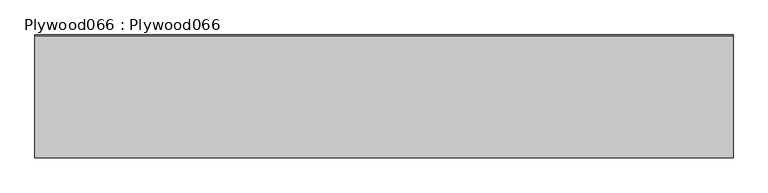
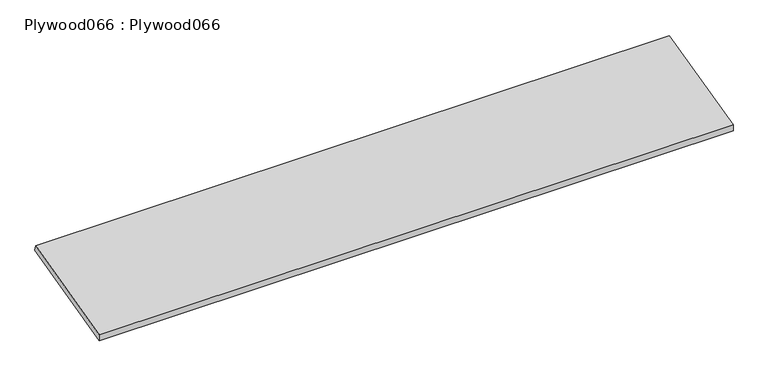
"""IFC4 building model written with IfcOpenShell, lengths in millimetres: proxy geometry, Plywood066 : Plywood066."""

from ifc_helpers import new_model, si_unit, frame, origin, place, context, project, spatial, polyline, outline, extrude, source, transform, mapped, element, save


def plywood066_plywood066_c0c2f735(model_context):
    return source(origin(), model_context, "Body", "SweptSolid", [
        extrude(outline(polyline([(10450.3071146, 43410.4220103), (10797.9696146, 43497.3618545), (10802.0009766, 43478.8789062), (10450.3071146, 43390.786725), (10450.3071146, 43410.4220103)])), frame((3694.0383192, 0.0, 0.0), z_axis=(1.0, 0.0, 0.0), x_axis=(0.0, 1.0, 0.0)), (0.0, 0.0, 1.0), 2000.25),
    ])


if __name__ == "__main__":
    model = new_model("IFC4")
    model_context = context("Model", 3, world=origin())
    ifc_project = project(units=[si_unit("LENGTHUNIT", "METRE", prefix="MILLI")], contexts=[model_context])
    site = spatial("IfcSite", under=ifc_project)
    building = spatial("IfcBuilding", under=site)
    placement = place(None, origin())
    plywood066_plywood066_shape = plywood066_plywood066_c0c2f735(model_context)
    element("IfcBuildingElementProxy", 1, Name="Plywood066 : Plywood066", ObjectType="Plywood066 : Plywood066", at=placement, inside=building, context=model_context, shape_type="MappedRepresentation", body=[
        mapped(plywood066_plywood066_shape, transform((0.0, 0.0, 0.0), x_axis=(1.0, 0.0, 0.0), y_axis=(0.0, 1.0, 0.0), z_axis=(0.0, 0.0, 1.0))),
    ])
    save(model, "model.ifc")

# Revit data of these elements
# Type "Plywood066 : Plywood066"
#   NameOverride = "Plywood066"
# Element 1 (IfcBuildingElementProxy, "Plywood066 : Plywood066")
#   Materials on its faces: "WHITE OAK (SPEC T.B.D.) OVER BUILDING WRAP"
# Materials
#   "WHITE OAK (SPEC T.B.D.) OVER BUILDING WRAP": class "Unassigned", colour RGB 227 188 136, transparency 0, Cost = 0
